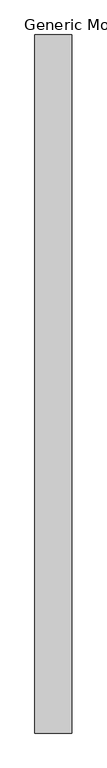
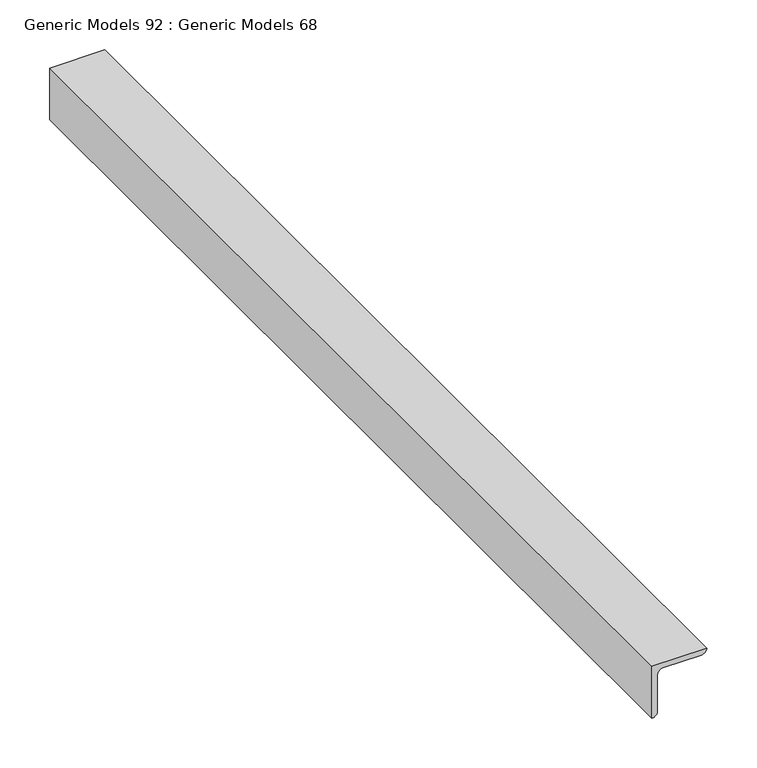
"""IFC4 building model written with IfcOpenShell, lengths in millimetres: proxy geometry, Generic Models 92 : Generic Models 68."""

from ifc_helpers import new_model, si_unit, point, frame, frame_2d, origin, place, context, project, spatial, polyline, circle_curve, trimmed, segment, composite_curve, outline, extrude, source, transform, mapped, element, save


def generic_models_92_generic_models_68_85783653(model_context):
    return source(origin(), model_context, "Body", "SweptSolid", [
        extrude(outline(composite_curve([segment(polyline([(266004.6986952, 20536.7616945), (265941.1986952, 20536.7616945)]), True, "CONTINUOUS"), segment(trimmed(circle_curve(frame_2d((265947.5486952, 20536.7616945)), 6.35), [point((265941.1986952, 20536.7616945))], [point((265947.5486952, 20543.1116945))], False, "CARTESIAN"), True, "CONTINUOUS"), segment(polyline([(265947.5486952, 20543.1116945), (265991.9986952, 20543.1116945)]), True, "CONTINUOUS"), segment(trimmed(circle_curve(frame_2d((265991.9986952, 20549.4616945)), 6.35), [point((265991.9986952, 20543.1116945))], [point((265998.3486952, 20549.4616945))], True, "CARTESIAN"), True, "CONTINUOUS"), segment(polyline([(265998.3486952, 20549.4616945), (265998.3486952, 20593.9116945)]), True, "CONTINUOUS"), segment(trimmed(circle_curve(frame_2d((266004.6986952, 20593.9116945)), 6.35), [point((265998.3486952, 20593.9116945))], [point((266004.6986952, 20600.2616945))], False, "CARTESIAN"), True, "CONTINUOUS"), segment(polyline([(266004.6986952, 20600.2616945), (266004.6986952, 20536.7616945)]), True, "CONTINUOUS")], self_intersect=False)), frame((0.0, 19721.5764581, 0.0), z_axis=(0.0, 1.0, 0.0), x_axis=(0.0, 0.0, 1.0)), (0.0, 0.0, 1.0), 1206.5),
    ])


if __name__ == "__main__":
    model = new_model("IFC4")
    model_context = context("Model", 3, world=origin())
    ifc_project = project(units=[si_unit("LENGTHUNIT", "METRE", prefix="MILLI")], contexts=[model_context])
    site = spatial("IfcSite", under=ifc_project)
    building = spatial("IfcBuilding", under=site)
    placement = place(None, origin())
    generic_models_92_generic_models_68_shape = generic_models_92_generic_models_68_85783653(model_context)
    element("IfcBuildingElementProxy", 1, Name="Generic Models 92 : Generic Models 68", ObjectType="Generic Models 92 : Generic Models 68", at=placement, inside=building, context=model_context, shape_type="MappedRepresentation", body=[
        mapped(generic_models_92_generic_models_68_shape, transform((0.0, 0.0, 0.0), x_axis=(1.0, 0.0, 0.0), y_axis=(0.0, 1.0, 0.0), z_axis=(0.0, 0.0, 1.0))),
    ])
    save(model, "model.ifc")

# Revit data of these elements
# Element 1 (IfcBuildingElementProxy, "Generic Models 92 : Generic Models 68")
#   Materials on its faces: "CAR DOOR RAIL: GALV. ANGLE L2 1/2 X 2 1/2 X 1/4\" @ 32\" ABOVE GRADE (PARALLEL TO HORTZ. WOOD TRIM)"
# Materials
#   "CAR DOOR RAIL: GALV. ANGLE L2 1/2 X 2 1/2 X 1/4\" @ 32\" ABOVE GRADE (PARALLEL TO HORTZ. WOOD TRIM)": class "Unassigned", colour RGB 211 211 211, transparency 0, Cost = 0
